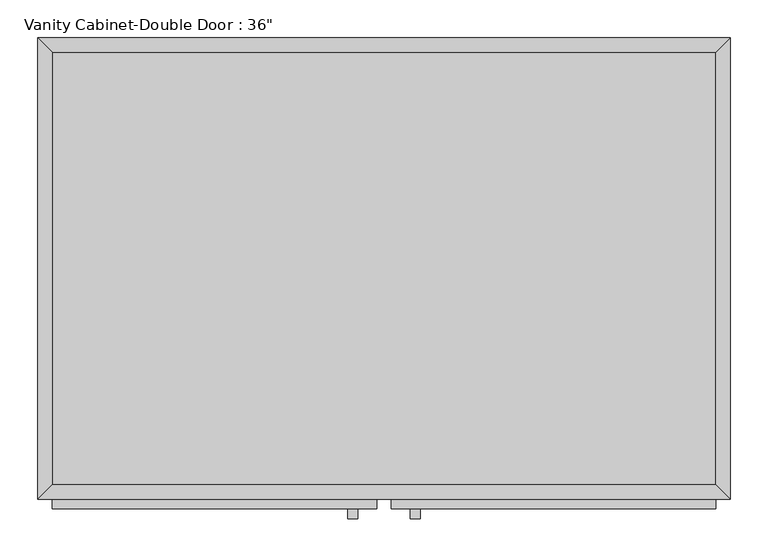
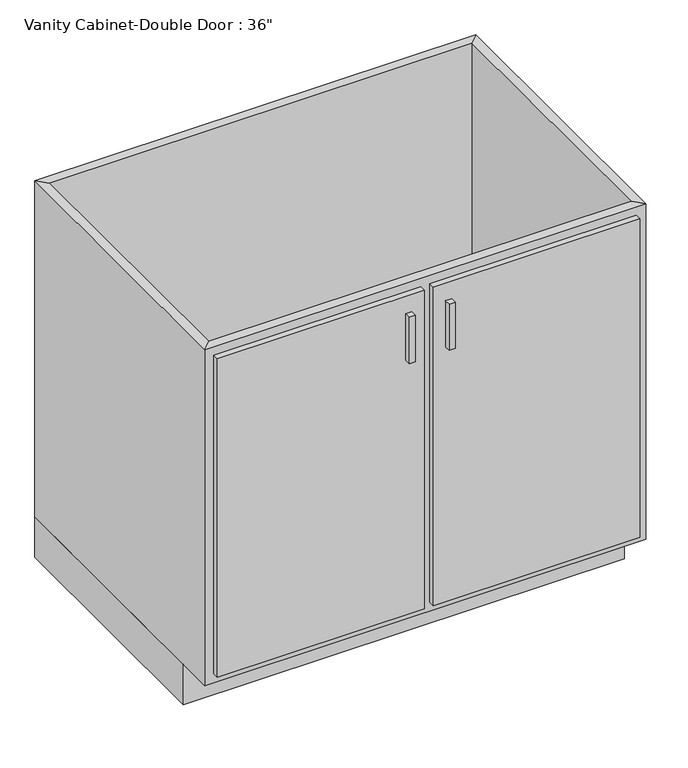
"""IFC4 building model written with IfcOpenShell, lengths in millimetres: furniture geometry."""

import ifcopenshell
import ifcopenshell.guid

model = None  # the IFC model being written
_history = None  # IfcOwnerHistory: only IFC2X3 demands one
_inside = {}  # id of a spatial element -> (the spatial element, [elements in it])
_under = {}  # id of a project, library or spatial element -> (it, [spatial elements below it])
_declared = {}  # id of a project -> (the project, [libraries it declares])
_typed = {}  # id of a type object -> (the type object, [elements of that type])
_made_of = {}  # id of a material, layer set ... -> (it, [elements and type objects made of it])


def new_model(schema):
    """Start an empty IFC model of exactly this schema.

    Asked for "IFC4X3", IfcOpenShell would pick the latest addendum, in which some entities
    have other attributes; the version numbers below select the first issue.
    IFC2X3 requires an IfcOwnerHistory on every rooted entity: one is made here for all.
    """
    global model, _history
    if schema == "IFC4X3":
        model = ifcopenshell.file(schema_version=(4, 3, 0, 0))
    else:
        model = ifcopenshell.file(schema=schema)
    _inside.clear()
    _under.clear()
    _declared.clear()
    _typed.clear()
    _made_of.clear()
    _history = None
    if model.schema == "IFC2X3":
        org = make("IfcOrganization", Name="unknown")
        user = make(
            "IfcPersonAndOrganization",
            ThePerson=make("IfcPerson", FamilyName="unknown"),
            TheOrganization=org,
        )
        app = make(
            "IfcApplication",
            ApplicationDeveloper=org,
            Version="unknown",
            ApplicationFullName="unknown",
            ApplicationIdentifier="unknown",
        )
        _history = make(
            "IfcOwnerHistory",
            OwningUser=user,
            OwningApplication=app,
            ChangeAction="ADDED",
            CreationDate=0,
        )
    return model


def make(cls, **values):
    """One entity of the class cls with the attributes given. An attribute that is None is left unset."""
    return model.create_entity(
        cls, **{name: value for name, value in values.items() if value is not None}
    )


def rooted(cls, **values):
    """An entity with a GlobalId (a new one), such as an element, a storey or a relation."""
    return make(cls, GlobalId=ifcopenshell.guid.new(), OwnerHistory=_history, **values)


def si_unit(unit_type, name, prefix=None):
    """IfcSIUnit, for example si_unit("LENGTHUNIT", "METRE", prefix="MILLI")."""
    return make("IfcSIUnit", UnitType=unit_type, Prefix=prefix, Name=name)


def assignment(units):
    """IfcUnitAssignment: the units of a project."""
    return None if units is None else make("IfcUnitAssignment", Units=units)


def point(xyz):
    """IfcCartesianPoint."""
    return None if xyz is None else make("IfcCartesianPoint", Coordinates=xyz)


def direction(xyz):
    """IfcDirection."""
    return None if xyz is None else make("IfcDirection", DirectionRatios=xyz)


def frame(location, z_axis=None, x_axis=None):
    """IfcAxis2Placement3D, a coordinate frame: its origin and axes. An axis left out is left unset."""
    return make(
        "IfcAxis2Placement3D",
        Location=point(location),
        Axis=direction(z_axis),
        RefDirection=direction(x_axis),
    )


def origin():
    """The frame at (0, 0, 0) with its axes left unset."""
    return frame((0.0, 0.0, 0.0))


def origin_with_axes():
    """The frame at (0, 0, 0) with the z axis (0, 0, 1) and the x axis (1, 0, 0) written out."""
    return frame((0.0, 0.0, 0.0), z_axis=(0.0, 0.0, 1.0), x_axis=(1.0, 0.0, 0.0))


def place(relative_to, where):
    """IfcLocalPlacement: puts the frame where relative to a parent placement (None: the world)."""
    return make(
        "IfcLocalPlacement", PlacementRelTo=relative_to, RelativePlacement=where
    )


def context(
    kind, dimensions, precision=None, world=None, true_north=None, identifier=None
):
    """IfcGeometricRepresentationContext, for example the 3D "Model" context."""
    return make(
        "IfcGeometricRepresentationContext",
        ContextIdentifier=identifier,
        ContextType=kind,
        CoordinateSpaceDimension=dimensions,
        Precision=precision,
        WorldCoordinateSystem=world,
        TrueNorth=true_north,
    )


def project(units=None, contexts=None):
    """IfcProject with its units and contexts."""
    return rooted(
        "IfcProject",
        Name="project",
        RepresentationContexts=contexts,
        UnitsInContext=assignment(units),
    )


def spatial(cls, under=None, at=None, **own):
    """A site, building, storey or space (cls), placed at a placement, below another one or the project."""
    s = rooted(cls, ObjectPlacement=at, **own)
    if under is not None:
        _under.setdefault(under.id(), (under, []))[1].append(s)
    return s


def polyline(points):
    """IfcPolyline through the points."""
    return make("IfcPolyline", Points=[point(p) for p in points])


def outline(outer, holes=None, kind="AREA"):
    """IfcArbitraryClosedProfileDef: a profile drawn as a closed curve; with holes, ...WithVoids."""
    if holes is None:
        return make("IfcArbitraryClosedProfileDef", ProfileType=kind, OuterCurve=outer)
    return make(
        "IfcArbitraryProfileDefWithVoids",
        ProfileType=kind,
        OuterCurve=outer,
        InnerCurves=holes,
    )


def extrude(swept, where, along, depth):
    """IfcExtrudedAreaSolid: the profile swept, set in the frame where, extruded along a direction by depth."""
    return make(
        "IfcExtrudedAreaSolid",
        SweptArea=swept,
        Position=where,
        ExtrudedDirection=direction(along),
        Depth=depth,
    )


def faces_of(points, faces, orient=None, outer=None):
    """IfcFace entities. A face is a list of loops; a loop is a list of indices into points, from 0.

    orient and outer hold one flag for each loop. By default every Orientation is true, the
    first loop of a face is its IfcFaceOuterBound and the others are IfcFaceBound.
    """
    made = []
    for i, loops in enumerate(faces):
        bounds = []
        for j, loop in enumerate(loops):
            is_outer = j == 0 if outer is None else outer[i][j]
            bounds.append(
                make(
                    "IfcFaceOuterBound" if is_outer else "IfcFaceBound",
                    Bound=make("IfcPolyLoop", Polygon=[points[k] for k in loop]),
                    Orientation=True if orient is None else orient[i][j],
                )
            )
        made.append(make("IfcFace", Bounds=bounds))
    return made


def faceted_brep(points, faces, orient=None, outer=None, voids=None):
    """IfcFacetedBrep: a solid bounded by flat faces; with voids (closed shells), ...WithVoids."""
    shared = [point(p) for p in points]
    hull = make("IfcClosedShell", CfsFaces=faces_of(shared, faces, orient, outer))
    if voids is None:
        return make("IfcFacetedBrep", Outer=hull)
    return make(
        "IfcFacetedBrepWithVoids",
        Outer=hull,
        Voids=[
            make(cls, CfsFaces=faces_of(shared, fs, o, b)) for cls, fs, o, b in voids
        ],
    )


def shape(context_of_items, identifier, shape_type, items):
    """IfcShapeRepresentation: the items that make up one representation, for example the "Body"."""
    return make(
        "IfcShapeRepresentation",
        ContextOfItems=context_of_items,
        RepresentationIdentifier=identifier,
        RepresentationType=shape_type,
        Items=items,
    )


def source(mapping_origin, context_of_items, identifier, shape_type, items):
    """IfcRepresentationMap: a shape defined once, which mapped items show again and again."""
    return make(
        "IfcRepresentationMap",
        MappingOrigin=mapping_origin,
        MappedRepresentation=shape(context_of_items, identifier, shape_type, items),
    )


def transform(
    local_origin,
    x_axis=None,
    y_axis=None,
    z_axis=None,
    scale=None,
    scale2=None,
    scale3=None,
    uniform=True,
):
    """IfcCartesianTransformationOperator3D, or its non-uniform kind. x_axis, y_axis, z_axis: its Axis1, 2, 3."""
    if uniform:
        return make(
            "IfcCartesianTransformationOperator3D",
            Axis1=direction(x_axis),
            Axis2=direction(y_axis),
            LocalOrigin=point(local_origin),
            Scale=scale,
            Axis3=direction(z_axis),
        )
    return make(
        "IfcCartesianTransformationOperator3DnonUniform",
        Axis1=direction(x_axis),
        Axis2=direction(y_axis),
        LocalOrigin=point(local_origin),
        Scale=scale,
        Axis3=direction(z_axis),
        Scale2=scale2,
        Scale3=scale3,
    )


def mapped(mapping_source, mapping_target):
    """IfcMappedItem: shows the shape of a source again, moved by a transform."""
    return make(
        "IfcMappedItem", MappingSource=mapping_source, MappingTarget=mapping_target
    )


def made_of(thing, what):
    """Note that an element or type object is made of a material, layer set ...; save() writes the relation."""
    if what is not None:
        _made_of.setdefault(what.id(), (what, []))[1].append(thing)
    return thing


def element(
    cls,
    number,
    at=None,
    inside=None,
    cuts=None,
    type_object=None,
    material=None,
    context=None,
    identifier="Body",
    shape_type=None,
    held_by="IfcProductDefinitionShape",
    body=None,
    shapes=None,
    **own,
):
    """One element of the class cls, such as IfcWall. Its Tag is "e" and its number.

    at: its placement. inside: the storey or other place that contains it. cuts: it is an
    opening in that element (IfcRelVoidsElement). A single representation is given by context,
    identifier, shape_type and body (its items); several are given by shapes. held_by: the class
    of the entity that holds the representations. save() writes the other relations.
    """
    e = rooted(cls, Tag="e%d" % number, ObjectPlacement=at, **own)
    if body is not None:
        shapes = [shape(context, identifier, shape_type, body)]
    if shapes is not None:
        e.Representation = make(held_by, Representations=shapes)
    if inside is not None:
        _inside.setdefault(inside.id(), (inside, []))[1].append(e)
    if cuts is not None:
        rooted(
            "IfcRelVoidsElement", RelatingBuildingElement=cuts, RelatedOpeningElement=e
        )
    if type_object is not None:
        _typed.setdefault(type_object.id(), (type_object, []))[1].append(e)
    return made_of(e, material)


def aggregate(whole, parts):
    """IfcRelAggregates: a whole, such as a stair, and the parts it consists of."""
    return rooted("IfcRelAggregates", RelatingObject=whole, RelatedObjects=parts)


def save(model, path):
    """Write the relations noted so far, then the file.

    IfcRelAggregates (storeys below a building ...), IfcRelContainedInSpatialStructure (elements
    in a storey), IfcRelDefinesByType, IfcRelAssociatesMaterial and IfcRelDeclares: one each for
    every whole, place, type object, material and project.
    """
    for whole, parts in _under.values():
        aggregate(whole, parts)
    for where, things in _inside.values():
        rooted(
            "IfcRelContainedInSpatialStructure",
            RelatedElements=things,
            RelatingStructure=where,
        )
    for kind, things in _typed.values():
        rooted("IfcRelDefinesByType", RelatedObjects=things, RelatingType=kind)
    for what, things in _made_of.values():
        rooted("IfcRelAssociatesMaterial", RelatedObjects=things, RelatingMaterial=what)
    for by, libraries in _declared.values():
        rooted("IfcRelDeclares", RelatingContext=by, RelatedDefinitions=libraries)
    model.write(path)


def furniture_828f600b(model_context):
    return source(origin(), model_context, "Body", "SolidModel", [
        extrude(outline(polyline([(-16.1872951, -635.0), (-28.8872951, -635.0), (-28.8872951, -622.3), (-16.1872951, -622.3), (-16.1872951, -635.0)])), frame((0.0, 0.0, 666.75), z_axis=(0.0, 0.0, 1.0), x_axis=(1.0, 0.0, 0.0)), (0.0, 0.0, 1.0), 101.6),
        extrude(outline(polyline([(66.3627049, -635.0), (53.6627049, -635.0), (53.6627049, -622.3), (66.3627049, -622.3), (66.3627049, -635.0)])), frame((0.0, 0.0, 666.75), z_axis=(0.0, 0.0, 1.0), x_axis=(1.0, 0.0, 0.0)), (0.0, 0.0, 1.0), 101.6),
        extrude(outline(polyline([(9.2127049, -622.3), (-419.4122951, -622.3), (-419.4122951, -609.6), (9.2127049, -609.6), (9.2127049, -622.3)])), frame((0.0, 0.0, 107.95), z_axis=(0.0, 0.0, 1.0), x_axis=(1.0, 0.0, 0.0)), (0.0, 0.0, 1.0), 698.5),
        extrude(outline(polyline([(456.8877049, -622.3), (28.2627049, -622.3), (28.2627049, -609.6), (456.8877049, -609.6), (456.8877049, -622.3)])), frame((0.0, 0.0, 107.95), z_axis=(0.0, 0.0, 1.0), x_axis=(1.0, 0.0, 0.0)), (0.0, 0.0, 1.0), 698.5),
        extrude(outline(polyline([(456.8877049, -19.05), (456.8877049, -590.55), (-419.4122951, -590.55), (-419.4122951, -19.05), (456.8877049, -19.05)])), frame((0.0, 0.0, 88.9), z_axis=(0.0, 0.0, 1.0), x_axis=(1.0, 0.0, 0.0)), (0.0, 0.0, 1.0), 19.05),
        faceted_brep([(456.8877049, -590.55, 825.5), (456.8877049, -590.55, 88.9), (-419.4122951, -590.55, 88.9), (-419.4122951, -590.55, 825.5), (475.9377049, -609.6, 825.5), (-438.4622951, -609.6, 825.5), (475.9377049, -609.6, 88.9), (-438.4622951, -609.6, 88.9), (-419.4122951, -19.05, 88.9), (-419.4122951, -19.05, 825.5), (-438.4622951, 0.0, 825.5), (-438.4622951, 0.0, 88.9), (456.8877049, -19.05, 88.9), (456.8877049, -19.05, 825.5), (475.9377049, 0.0, 825.5), (475.9377049, 0.0, 88.9)], [[[0, 1, 2, 3]], [[4, 0, 3, 5]], [[6, 4, 5, 7]], [[1, 6, 7, 2]], [[3, 2, 8, 9]], [[5, 3, 9, 10]], [[7, 5, 10, 11]], [[2, 7, 11, 8]], [[9, 8, 12, 13]], [[10, 9, 13, 14]], [[11, 10, 14, 15]], [[8, 11, 15, 12]], [[13, 12, 1, 0]], [[14, 13, 0, 4]], [[15, 14, 4, 6]], [[12, 15, 6, 1]]]),
        extrude(outline(polyline([(475.9377049, 0.0), (475.9377049, -533.4), (-438.4622951, -533.4), (-438.4622951, 0.0), (475.9377049, 0.0)])), origin_with_axes(), (0.0, 0.0, 1.0), 88.9),
    ])


if __name__ == "__main__":
    model = new_model("IFC4")
    model_context = context("Model", 3, world=origin())
    ifc_project = project(units=[si_unit("LENGTHUNIT", "METRE", prefix="MILLI")], contexts=[model_context])
    site = spatial("IfcSite", under=ifc_project)
    building = spatial("IfcBuilding", under=site)
    placement = place(None, origin())
    furniture_shape = furniture_828f600b(model_context)
    element("IfcFurniture", 1, ObjectType="Vanity Cabinet-Double Door : 36\"", at=placement, inside=building, context=model_context, shape_type="MappedRepresentation", body=[
        mapped(furniture_shape, transform((0.0, 0.0, 0.0), x_axis=(1.0, 0.0, 0.0), y_axis=(0.0, 1.0, 0.0), z_axis=(0.0, 0.0, 1.0))),
    ])
    save(model, "model.ifc")

# Revit data of these elements
# Type "Vanity Cabinet-Double Door : 36\""
#   Finish = "Cabinetry"
#   Finish = "Cabinetry"
#   Assembly Code = "C1030410"
#   Depth = 2' - 0"
#   Height = 2' - 8 1/2"
#   Toe Depth = 0' - 3"
#   Toe Height = 0' - 3 1/2"
#   Width = 3' - 0"
#   Cabinet Material = none
#   Door/Drawer Material = none
#   Handle Material = none
# Element 1 (IfcFurniture, "Vanity Cabinet-Double Door : 36\"")
#   Materials on its faces: "CASEWORK"
# Materials
#   "CASEWORK": class "Generic", colour RGB 181 181 181, transparency 0, Cost = 0
